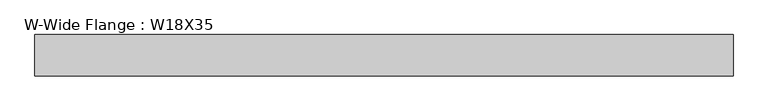
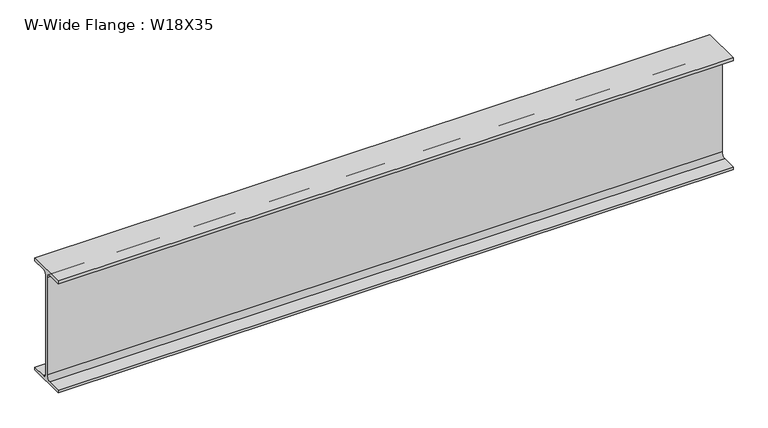
"""IFC4 building model written with IfcOpenShell, lengths in millimetres: beam geometry, W-Wide Flange : W18X35."""

from ifc_helpers import new_model, si_unit, point, frame, frame_2d, origin, place, context, project, spatial, polyline, circle_curve, trimmed, segment, composite_curve, outline, extrude, source, transform, mapped, element, save


def w_wide_flange_w18x35_15206e23(model_context):
    return source(origin(), model_context, "Body", "SweptSolid", [
        extrude(outline(composite_curve([segment(polyline([(76.2, -213.995), (76.2, -224.79), (-76.2, -224.79), (-76.2, -213.995), (-21.59, -213.995)]), True, "CONTINUOUS"), segment(trimmed(circle_curve(frame_2d((-21.59, -196.215)), 17.78), [point((-21.59, -213.995))], [point((-3.81, -196.215))], True, "CARTESIAN"), True, "CONTINUOUS"), segment(polyline([(-3.81, -196.215), (-3.81, 196.215)]), True, "CONTINUOUS"), segment(trimmed(circle_curve(frame_2d((-21.59, 196.215)), 17.78), [point((-3.81, 196.215))], [point((-21.59, 213.995))], True, "CARTESIAN"), True, "CONTINUOUS"), segment(polyline([(-21.59, 213.995), (-76.2, 213.995), (-76.2, 224.79), (76.2, 224.79), (76.2, 213.995), (21.59, 213.995)]), True, "CONTINUOUS"), segment(trimmed(circle_curve(frame_2d((21.59, 196.215)), 17.78), [point((21.59, 213.995))], [point((3.81, 196.215))], True, "CARTESIAN"), True, "CONTINUOUS"), segment(polyline([(3.81, 196.215), (3.81, -196.215)]), True, "CONTINUOUS"), segment(trimmed(circle_curve(frame_2d((21.59, -196.215)), 17.78), [point((3.81, -196.215))], [point((21.59, -213.995))], True, "CARTESIAN"), True, "CONTINUOUS"), segment(polyline([(21.59, -213.995), (76.2, -213.995)]), True, "CONTINUOUS")], self_intersect=False)), frame((-1282.7, 0.0, 0.0), z_axis=(1.0, 0.0, 0.0), x_axis=(0.0, 1.0, 0.0)), (0.0, 0.0, 1.0), 2565.4),
    ])


if __name__ == "__main__":
    model = new_model("IFC4")
    model_context = context("Model", 3, world=origin())
    ifc_project = project(units=[si_unit("LENGTHUNIT", "METRE", prefix="MILLI")], contexts=[model_context])
    site = spatial("IfcSite", under=ifc_project)
    building = spatial("IfcBuilding", under=site)
    placement = place(None, origin())
    w_wide_flange_w18x35_shape = w_wide_flange_w18x35_15206e23(model_context)
    element("IfcBeam", 1, ObjectType="W-Wide Flange : W18X35", at=placement, inside=building, context=model_context, shape_type="MappedRepresentation", body=[
        mapped(w_wide_flange_w18x35_shape, transform((0.0, 0.0, 0.0), x_axis=(1.0, 0.0, 0.0), y_axis=(0.0, 1.0, 0.0), z_axis=(0.0, 0.0, 1.0))),
    ])
    save(model, "model.ifc")

# Revit data of these elements
# Type "W-Wide Flange : W18X35"
#   Assembly Code = "B10"
#   W = 35
#   Length [instance default] = 5' - 0"
#   bf = 0' - 6"
#   d = 1' - 5.7"
#   k = 0' - 1 1/8"
#   k2 = 0' - 0.7"
#   tf = 0' - 0.425"
#   tw = 0' - 0.3"
#   A = 0.0715278 SF
#   Structural Material [instance default] = Steel ASTM A992
# Element 1 (IfcBeam, "W-Wide Flange : W18X35")
#   Materials on its faces: "Steel ASTM A992"
# Materials
#   "Steel ASTM A992": class "Metal", colour RGB 199 199 199, transparency 0, Description = "Structural steel 50ksi", Cost = 0
